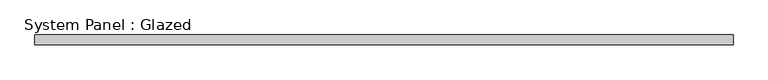
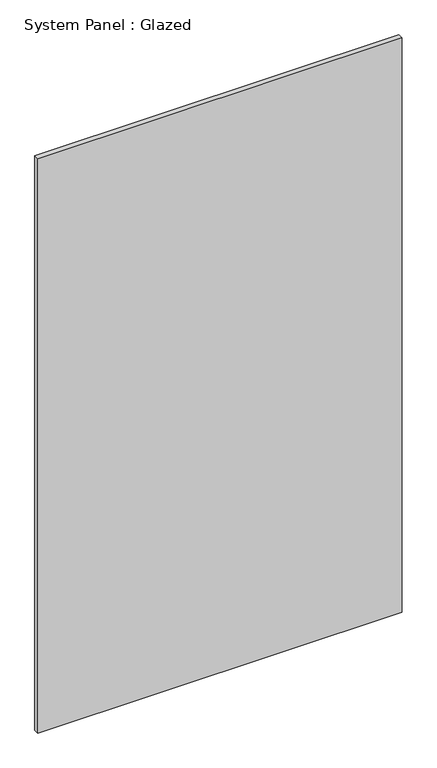
"""IFC4 building model written with IfcOpenShell, lengths in millimetres: plate geometry, System Panel : Glazed."""

from ifc_helpers import new_model, si_unit, origin, origin_with_axes, place, context, project, spatial, polyline, outline, extrude, source, transform, mapped, element, save


def system_panel_glazed_bff502fa(model_context):
    return source(origin(), model_context, "Body", "SweptSolid", [
        extrude(outline(polyline([(914.4000002, 19.05), (-914.4000002, 19.05), (-914.4000002, 44.45), (914.4000002, 44.45), (914.4000002, 19.05)])), origin_with_axes(), (0.0, 0.0, 1.0), 3048.0),
    ])


if __name__ == "__main__":
    model = new_model("IFC4")
    model_context = context("Model", 3, world=origin())
    ifc_project = project(units=[si_unit("LENGTHUNIT", "METRE", prefix="MILLI")], contexts=[model_context])
    site = spatial("IfcSite", under=ifc_project)
    building = spatial("IfcBuilding", under=site)
    placement = place(None, origin())
    system_panel_glazed_shape = system_panel_glazed_bff502fa(model_context)
    element("IfcPlate", 1, ObjectType="System Panel : Glazed", at=placement, inside=building, context=model_context, shape_type="MappedRepresentation", body=[
        mapped(system_panel_glazed_shape, transform((0.0, 0.0, 0.0), x_axis=(1.0, 0.0, 0.0), y_axis=(0.0, 1.0, 0.0), z_axis=(0.0, 0.0, 1.0))),
    ])
    save(model, "model.ifc")

# Revit data of these elements
# Type "System Panel : Glazed"
#   Construction Type Id = "GSP4R"
#   Analytic Construction = "1/8 in Pilkington single glazing"
#   Visual Light Transmittance = 0.9
#   Solar Heat Gain Coefficient = 0.86
#   Heat Transfer Coefficient (U) = 1.18115 BTU/(h·ft²·°F)
#   Define Thermal Properties by = 1
# Element 1 (IfcPlate, "System Panel : Glazed")
#   Materials on its faces: "Glass"
# Materials
#   "Glass": class "Glass", colour RGB 0 128 192, transparency 0.75, Description = "Soda Lime Glass", Cost = 0
